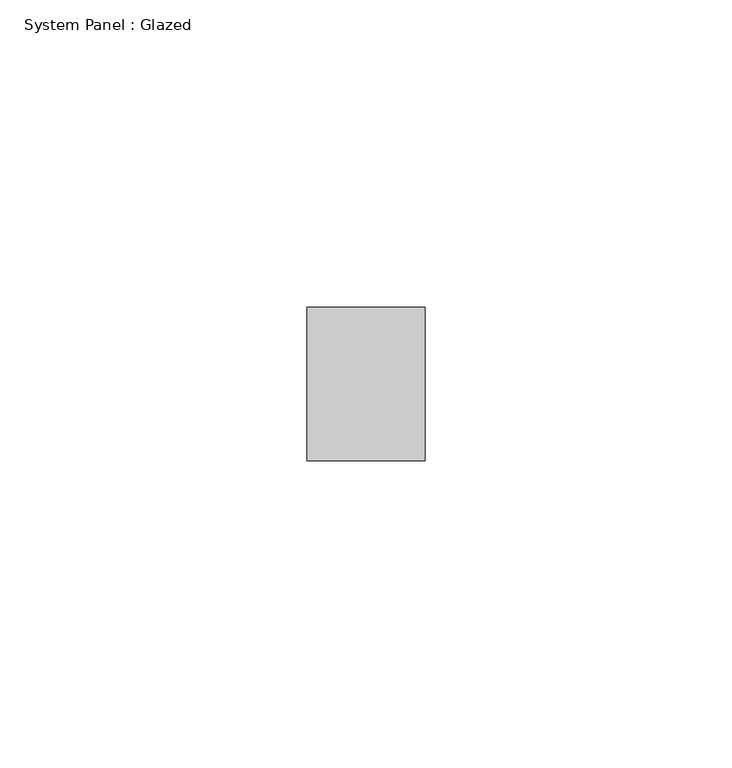
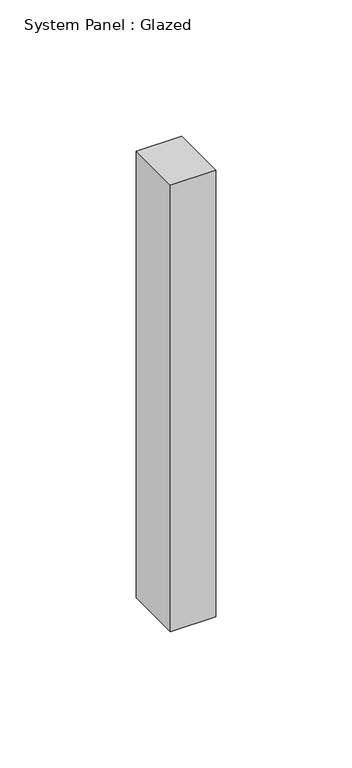
"""IFC4 building model written with IfcOpenShell, lengths in millimetres: plate geometry, System Panel : Glazed."""

from ifc_helpers import new_model, si_unit, origin, origin_with_axes, place, context, project, spatial, polyline, outline, extrude, source, transform, mapped, element, save


def system_panel_glazed_1102e745(model_context):
    return source(origin(), model_context, "Body", "SweptSolid", [
        extrude(outline(polyline([(9.6033902, 24.5), (-9.6033902, 24.5), (-9.6033902, 49.5), (9.6033902, 49.5), (9.6033902, 24.5)])), origin_with_axes(), (0.0, 0.0, 1.0), 200.0),
    ])


if __name__ == "__main__":
    model = new_model("IFC4")
    model_context = context("Model", 3, world=origin())
    ifc_project = project(units=[si_unit("LENGTHUNIT", "METRE", prefix="MILLI")], contexts=[model_context])
    site = spatial("IfcSite", under=ifc_project)
    building = spatial("IfcBuilding", under=site)
    placement = place(None, origin())
    system_panel_glazed_shape = system_panel_glazed_1102e745(model_context)
    element("IfcPlate", 1, ObjectType="System Panel : Glazed", at=placement, inside=building, context=model_context, shape_type="MappedRepresentation", body=[
        mapped(system_panel_glazed_shape, transform((0.0, 0.0, 0.0), x_axis=(1.0, 0.0, 0.0), y_axis=(0.0, 1.0, 0.0), z_axis=(0.0, 0.0, 1.0))),
    ])
    save(model, "model.ifc")

# Revit data of these elements
# Element 1 (IfcPlate, "System Panel : Glazed")
#   Materials on its faces: "Glass"
# Materials
#   "Glass": class "Glass", colour RGB 218 227 224, transparency 0.85, Description = "Soda Lime Glass", Cost = 0
